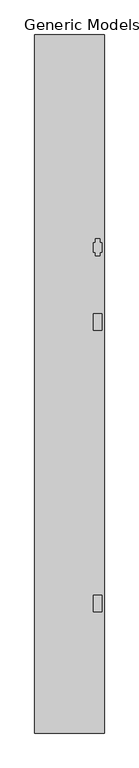
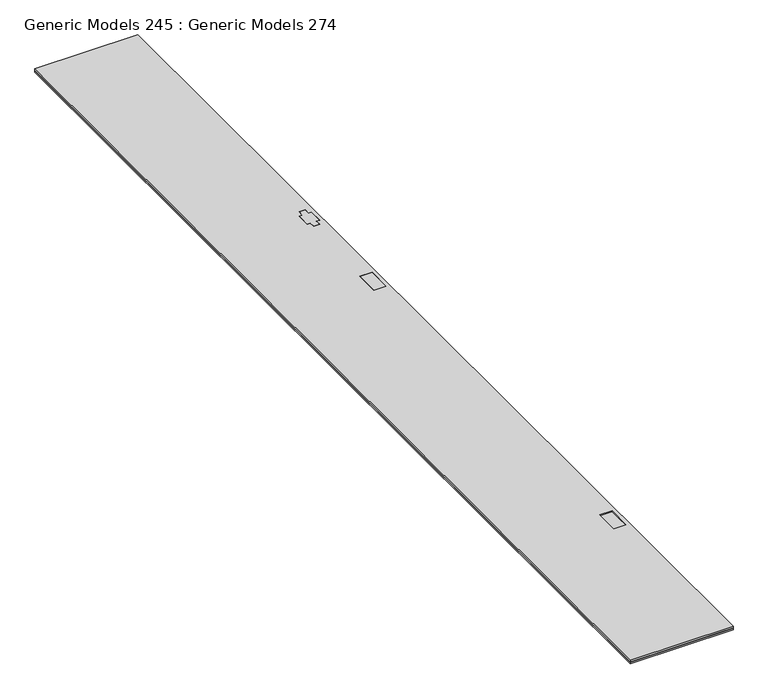
"""IFC4 building model written with IfcOpenShell, lengths in millimetres: proxy geometry, Generic Models 245 : Generic Models 274."""

from ifc_helpers import new_model, si_unit, frame, origin, place, context, project, spatial, polyline, outline, extrude, source, transform, mapped, element, save


def generic_models_245_generic_models_274_214f66cd(model_context):
    return source(origin(), model_context, "Body", "SweptSolid", [
        extrude(outline(polyline([(32019.8715778, 36483.6207942), (32053.2090778, 36483.6207942), (32053.2090778, 36331.2207942), (32019.8715778, 36331.2207942), (32019.8715778, 36274.0707942), (31956.3715778, 36274.0707942), (31956.3715778, 36331.2207942), (31923.0340778, 36331.2207942), (31923.0340778, 36483.6207942), (31956.3715778, 36483.6207942), (31956.3715778, 36540.7707942), (32019.8715778, 36540.7707942), (32019.8715778, 36483.6207942)])), frame((0.0, 0.0, 266376.15), z_axis=(0.0, 0.0, 1.0), x_axis=(1.0, 0.0, 0.0)), (0.0, 0.0, 1.0), 38.1),
        extrude(outline(polyline([(32091.3210525, 39739.741111), (32091.3210525, 28794.1408334), (30999.1210525, 28794.1408334), (30999.1210525, 39739.741111), (32091.3210525, 39739.741111)]), holes=[polyline([(31923.0340778, 36274.0707942), (32053.2090778, 36274.0707942), (32053.2090778, 36540.7707942), (31923.0340778, 36540.7707942), (31923.0340778, 36274.0707942)]), polyline([(31923.0340778, 35112.0207942), (32053.2090778, 35112.0207942), (32053.2090778, 35366.0207942), (31923.0340778, 35366.0207942), (31923.0340778, 35112.0207942)]), polyline([(31923.0340778, 30698.1406612), (32053.2090778, 30698.1406612), (32053.2090778, 30952.1406612), (31923.0340778, 30952.1406612), (31923.0340778, 30698.1406612)])]), frame((0.0, 0.0, 266376.15), z_axis=(0.0, 0.0, 1.0), x_axis=(1.0, 0.0, 0.0)), (0.0, 0.0, 1.0), 19.05),
        extrude(outline(polyline([(32053.2090778, 30952.1406612), (32053.2090778, 30698.1406612), (31923.0340778, 30698.1406612), (31923.0340778, 30952.1406612), (32053.2090778, 30952.1406612)])), frame((0.0, 0.0, 266376.15), z_axis=(0.0, 0.0, 1.0), x_axis=(1.0, 0.0, 0.0)), (0.0, 0.0, 1.0), 28.8734047),
        extrude(outline(polyline([(32053.2090778, 35366.0207942), (32053.2090778, 35112.0207942), (31923.0340778, 35112.0207942), (31923.0340778, 35366.0207942), (32053.2090778, 35366.0207942)])), frame((0.0, 0.0, 266376.15), z_axis=(0.0, 0.0, 1.0), x_axis=(1.0, 0.0, 0.0)), (0.0, 0.0, 1.0), 38.1),
        extrude(outline(polyline([(32091.3210525, 39739.741111), (32091.3210525, 28794.1408334), (30999.1210525, 28794.1408334), (30999.1210525, 39739.741111), (32091.3210525, 39739.741111)]), holes=[polyline([(31923.0340778, 35112.0207942), (32053.2090778, 35112.0207942), (32053.2090778, 35366.0207942), (31923.0340778, 35366.0207942), (31923.0340778, 35112.0207942)]), polyline([(31923.0340778, 30698.1406612), (32053.2090778, 30698.1406612), (32053.2090778, 30952.1406612), (31923.0340778, 30952.1406612), (31923.0340778, 30698.1406612)]), polyline([(31923.0340778, 36331.2207942), (31956.3715778, 36331.2207942), (31956.3715778, 36274.0707942), (32019.8715778, 36274.0707942), (32019.8715778, 36331.2207942), (32053.2090778, 36331.2207942), (32053.2090778, 36483.6207942), (32019.8715778, 36483.6207942), (32019.8715778, 36540.7707942), (31956.3715778, 36540.7707942), (31956.3715778, 36483.6207942), (31923.0340778, 36483.6207942), (31923.0340778, 36331.2207942)])]), frame((0.0, 0.0, 266395.2), z_axis=(0.0, 0.0, 1.0), x_axis=(1.0, 0.0, 0.0)), (0.0, 0.0, 1.0), 19.05),
    ])


if __name__ == "__main__":
    model = new_model("IFC4")
    model_context = context("Model", 3, world=origin())
    ifc_project = project(units=[si_unit("LENGTHUNIT", "METRE", prefix="MILLI")], contexts=[model_context])
    site = spatial("IfcSite", under=ifc_project)
    building = spatial("IfcBuilding", under=site)
    placement = place(None, origin())
    generic_models_245_generic_models_274_shape = generic_models_245_generic_models_274_214f66cd(model_context)
    element("IfcBuildingElementProxy", 1, Name="Generic Models 245 : Generic Models 274", ObjectType="Generic Models 245 : Generic Models 274", at=placement, inside=building, context=model_context, shape_type="MappedRepresentation", body=[
        mapped(generic_models_245_generic_models_274_shape, transform((0.0, 0.0, 0.0), x_axis=(1.0, 0.0, 0.0), y_axis=(0.0, 1.0, 0.0), z_axis=(0.0, 0.0, 1.0))),
    ])
    save(model, "model.ifc")

# Revit data of these elements
# Element 1 (IfcBuildingElementProxy, "Generic Models 245 : Generic Models 274")
#   Materials on its faces: "TREATED BLOCKING AT NECESSARY TO BRING UP TO FINISH FLOOR ELEV.", "HARD WOOD FLOOR", "3/4\" PRESSURE TREATED CDX PLYWOOD"
# Materials
#   "TREATED BLOCKING AT NECESSARY TO BRING UP TO FINISH FLOOR ELEV.": class "Wood", colour RGB 144 113 62, transparency 0, Description = "Pinus Echinata", Cost = 0
#   "HARD WOOD FLOOR": class "Wood", colour RGB 166 116 52, transparency 0, Cost = 0
#   "3/4\" PRESSURE TREATED CDX PLYWOOD": class "Wood", colour RGB 144 113 62, transparency 0, Description = "Pinus Echinata", Cost = 0
